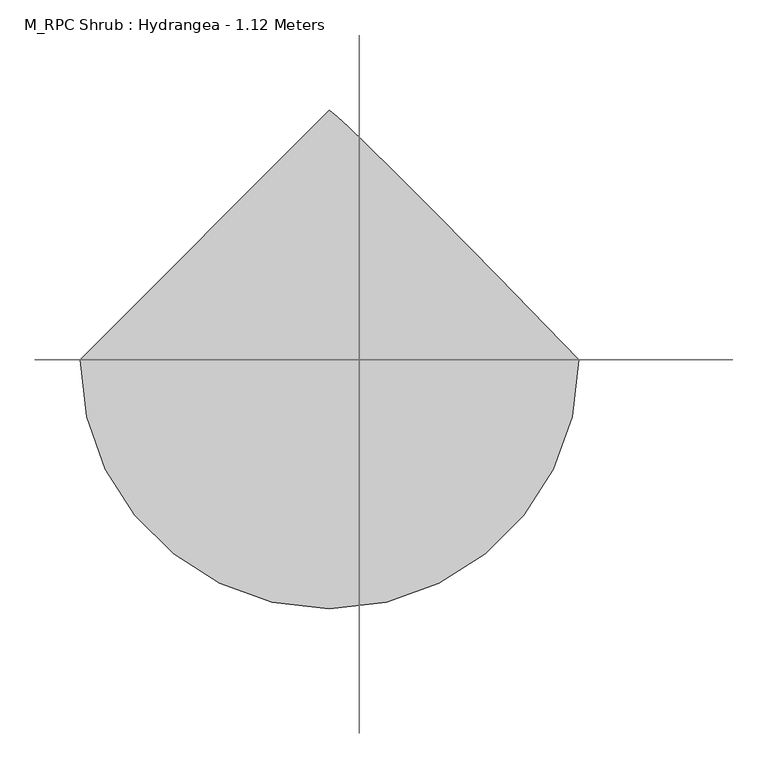
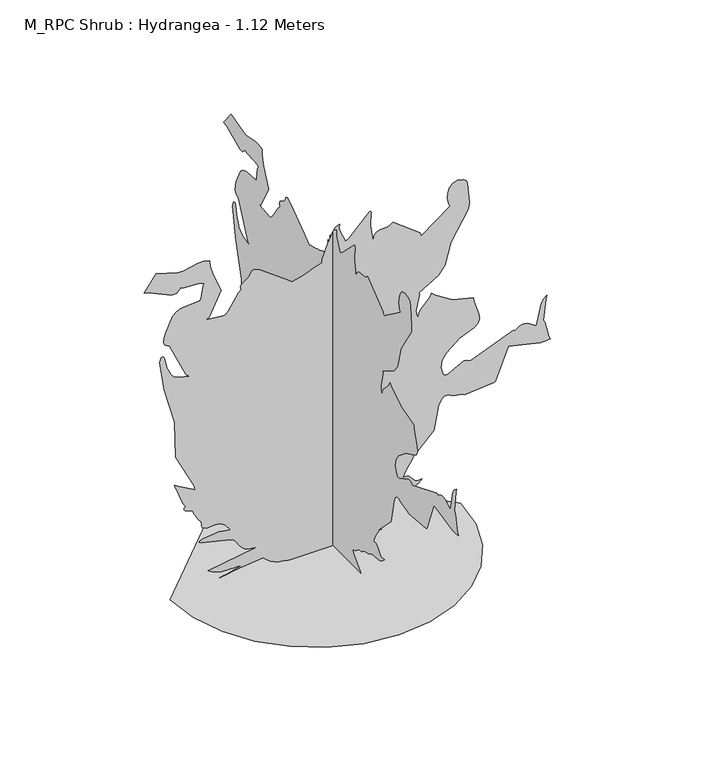
"""IFC4 building model written with IfcOpenShell, lengths in millimetres: geographic element geometry, M_RPC Shrub : Hydrangea - 1.12 Meters."""

from ifc_helpers import new_model, si_unit, origin, place, context, project, spatial, triangles, source, transform, mapped, element, save


def m_rpc_shrub_hydrangea_1_12_meters_e26dcdf9(model_context):
    return source(origin(), model_context, "Body", "Tessellation", [
        triangles([(-465.7652839, 0.0, 3.03e-05), (-453.4503742, -106.722383, 3.03e-05), (-418.3841643, -204.7301452, 3.03e-05), (-363.3691721, -291.2156366, 3.03e-05), (-291.2156366, -363.3691721, 3.03e-05), (-204.7298909, -418.3841643, 3.03e-05), (-106.722383, -453.4503742, 3.03e-05), (2.04e-05, -465.7652839, 3.03e-05), (106.7226373, -453.4503742, 3.03e-05), (204.7301452, -418.3841643, 3.03e-05), (291.2156366, -363.3691721, 3.03e-05), (363.3691721, -291.2156366, 3.03e-05), (418.3841643, -204.7298909, 3.03e-05), (453.4503742, -106.722383, 3.03e-05), (465.7652839, 4.07e-05, 3.03e-05), (314.4022119, 155.2617258, 3.03e-05), (202.1882401, 269.5741523, 3.03e-05), (122.6004381, 349.7611364, 3.03e-05), (69.1127373, 402.650677, 3.03e-05), (35.2001157, 435.0619981, 3.03e-05), (14.3374424, 453.8270954, 3.03e-05), (-6.11e-05, 465.7652839, 3.03e-05), (56.1492344, -378.5859032, 896.584009), (56.1492344, -435.8001798, 990.1474113), (56.1492344, -437.9638195, 1010.0427086), (56.1492344, -432.6209044, 1076.3849527), (56.1492344, -428.4870724, 1086.8671618), (56.1492344, -421.1205162, 1093.7984247), (56.1492344, -400.1306637, 1098.3878975), (56.1492344, -384.9139326, 1093.7296789), (56.1492344, -374.9204656, 1082.3183842), (56.1492344, -369.6029849, 1066.6409254), (56.1492344, -368.4091624, 1049.1918451), (56.1492344, -370.7917205, 1032.4579828), (56.1492344, -376.200838, 1018.9314102), (56.1492344, -284.4905202, 951.5531828), (56.1492344, -279.0483378, 962.8982752), (56.1492344, -192.4284615, 1029.6936167), (56.1492344, -183.9065071, 1021.5888788), (56.1492344, -173.6880356, 1018.7583103), (56.1492344, -151.8174592, 1018.2594309), (56.1492344, -141.9947939, 1015.253219), (56.1492344, -134.1316202, 1006.853223), (56.1492344, -129.1432891, 990.3891844), (56.1492344, -120.5388725, 1040.242028), (56.1492344, -122.2206557, 1090.0057056), (56.1492344, -121.588872, 1091.2198757), (56.1492344, -120.5788409, 1091.6016838), (56.1492344, -119.3498916, 1091.314056), (56.1492344, -118.0631606, 1090.5223892), (56.1492344, -51.1270437, 1024.7248793), (56.1492344, -40.2401219, 1017.5288795), (56.1492344, -21.4382513, 1061.8860558), (56.1492344, -19.9459255, 1071.2685499), (56.1492344, -20.5882464, 1082.5678602), (56.1492344, -9.2161605, 1076.7642174), (56.1492344, -0.541737, 1066.0147282), (56.1492344, 13.2312884, 1034.0107224), (56.1492344, 15.0516987, 1033.3972424), (56.1492344, 16.1430633, 1042.7950699), (56.1492344, 15.8630375, 1032.315477), (56.1492344, 35.0076788, 982.2768162), (56.1492344, 34.7279334, 971.7971506), (56.1492344, 47.0023863, 967.7320644), (56.1492344, 59.9819265, 963.0433245), (56.1492344, 73.5461604, 958.0542395), (56.1492344, 87.5764677, 953.090589), (56.1492344, 101.9527068, 948.4782251), (56.1492344, 116.5559942, 944.5379133), (56.1492344, 131.266706, 941.5953604), (56.1492344, 159.1710257, 963.3564594), (56.1492344, 234.8070158, 1017.7426746), (56.1492344, 253.0856966, 1025.9415928), (56.1492344, 261.255583, 1022.6172318), (56.1492344, 265.0508637, 1010.9616205), (56.1492344, 271.5392395, 1003.587434), (56.1492344, 292.8116329, 989.8291895), (56.1492344, 295.7185412, 982.2462948), (56.1492344, 294.1403672, 970.2699183), (56.1492344, 302.2043736, 963.0229769), (56.1492344, 334.2949656, 913.7683525), (56.1492344, 342.6898747, 905.5160219), (56.1492344, 351.4004259, 902.5404041), (56.1492344, 406.148138, 908.504357), (56.1492344, 397.9441329, 914.2774784), (56.1492344, 358.0695319, 991.6771872), (56.1492344, 384.2062723, 1053.5038639), (56.1492344, 393.7135772, 1085.5969631), (56.1492344, 394.9175735, 1105.0289892), (56.1492344, 414.6906761, 1109.8475178), (56.1492344, 432.1779808, 1109.2748056), (56.1492344, 480.121675, 1098.4515564), (56.1492344, 497.6624285, 1099.5588289), (56.1492344, 567.1076082, 1120.0013311), (56.1492344, 606.4145476, 1067.5955183), (56.1492344, 591.7069061, 1065.4878708), (56.1492344, 517.0715272, 1030.4623198), (56.1492344, 500.9715288, 1032.2518181), (56.1492344, 488.49878, 1045.1369328), (56.1492344, 477.9249341, 1041.5376612), (56.1492344, 432.2085385, 1040.0638412), (56.1492344, 422.1870572, 1037.8874479), (56.1492344, 413.6343089, 1032.9696522), (56.1492344, 417.3048697, 1026.0867147), (56.1492344, 423.0626942, 986.5124588), (56.1492344, 426.7357985, 979.6269779), (56.1492344, 479.2129369, 976.8397207), (56.1492344, 491.6474977, 973.836125), (56.1492344, 503.2929714, 967.8211578), (56.1492344, 513.8846214, 957.7538944), (56.1492344, 537.5548336, 908.2956488), (56.1492344, 541.9203012, 892.3381926), (56.1492344, 542.610121, 878.2821465), (56.1492344, 538.0995678, 867.797394), (56.1492344, 524.5653648, 859.2141243), (56.1492344, 471.3347477, 744.5693052), (56.1492344, 460.1321975, 735.9044998), (56.1492344, 496.5424387, 744.6049135), (56.1492344, 507.3555141, 749.4158117), (56.1492344, 516.4402794, 756.3470747), (56.1492344, 523.1577473, 766.0961889), (56.1492344, 526.8690033, 779.3631117), (56.1492344, 532.2882946, 786.419149), (56.1492344, 540.9835851, 826.8283104), (56.1492344, 544.9977659, 831.6620996), (56.1492344, 551.7839433, 831.0664965), (56.1492344, 556.8366872, 815.0530117), (56.1492344, 541.9737499, 718.1015894), (56.1492344, 508.528989, 595.9425488), (56.1492344, 504.1736953, 476.8583931), (56.1492344, 445.00198, 359.8157189), (56.1492344, 442.0517967, 344.7389503), (56.1492344, 498.367509, 375.5670104), (56.1492344, 507.2155154, 382.5721061), (56.1492344, 508.4017076, 380.6935507), (56.1492344, 480.3736945, 310.0265705), (56.1492344, 472.5896856, 298.8163718), (56.1492344, 477.8714853, 294.0410819), (56.1492344, 477.8587681, 289.3930734), (56.1492344, 474.0736794, 285.1268912), (56.1492344, 461.2776581, 278.7937931), (56.1492344, 455.3060022, 277.2436152), (56.1492344, 451.6507384, 277.1188771), (56.1492344, 448.9347342, 271.42215), (56.1492344, 446.3994601, 265.944323), (56.1492344, 443.8616426, 260.5352237), (56.1492344, 441.1354646, 255.0446795), (56.1492344, 438.0401593, 249.3240076), (56.1492344, 434.3950693, 243.2202559), (56.1492344, 430.0117976, 236.5850141), (56.1492344, 424.8445258, 231.9143507), (56.1492344, 422.1564995, 227.0286025), (56.1492344, 421.13069, 222.1354782), (56.1492344, 420.9550467, 217.4424143), (56.1492344, 420.8125045, 213.1568838), (56.1492344, 419.8910491, 209.4863229), (56.1492344, 417.376159, 206.6384771), (56.1492344, 405.2165088, 201.5623153), (56.1492344, 393.8230182, 201.2377712), (56.1492344, 382.6001204, 202.7596986), (56.1492344, 370.95719, 203.2227154), (56.1492344, 358.2935371, 199.7216937), (56.1492344, 344.018609, 189.3512511), (56.1492344, 327.5393097, 169.2057329), (56.1492344, 364.5146327, 175.1936668), (56.1492344, 416.1365181, 169.3225681), (56.1492344, 425.6743443, 165.5346816), (56.1492344, 428.6066872, 161.7190351), (56.1492344, 423.5107046, 158.722016), (56.1492344, 327.5393097, 135.5160923), (56.1492344, 317.0469269, 128.8205254), (56.1492344, 309.0694705, 119.4107255), (56.1492344, 301.848, 108.7037664), (56.1492344, 293.6134553, 98.116195), (56.1492344, 282.5992476, 89.0650578), (56.1492344, 267.0465086, 82.9669016), (56.1492344, 245.1858699, 81.2382826), (56.1492344, 400.5328557, 55.0353398), (56.1492344, 387.9633831, 46.5487848), (56.1492344, 359.4237007, 37.5090999), (56.1492344, 291.9767275, 36.3188451), (56.1492344, 338.6400493, 23.9801451), (56.1492344, 350.1684154, 21.3613778), (56.1492344, 363.0993484, 18.5382114), (56.1492344, 356.3946342, 19.4966274), (56.1492344, 339.2585798, 22.5081329), (56.1492344, 315.3211238, 26.7056692), (56.1492344, 224.2112962, 38.0176831), (56.1492344, 212.000995, 26.2095603), (56.1492344, 199.2024303, 17.3446467), (56.1492344, 185.91387, 10.9324609), (56.1492344, 172.2333097, 6.482364), (56.1492344, 158.2584905, 3.5041026), (56.1492344, 144.0879256, 1.5067812), (56.1492344, 129.8191018, 0.0), (56.1492344, -156.6362603, 8.5e-06), (56.1492344, -151.989787, 6.9042229), (56.1492344, -116.5554855, 39.0040464), (56.1492344, -111.7351584, 47.433074), (56.1492344, -111.8306104, 55.7371229), (56.1492344, -119.5942535, 57.0004315), (56.1492344, -125.4931031, 59.6629825), (56.1492344, -130.4834689, 63.2543694), (56.1492344, -135.5219514, 67.303936), (56.1492344, -141.5656232, 71.3410306), (56.1492344, -149.5703308, 74.8950015), (56.1492344, -160.4934013, 77.495188), (56.1492344, -169.3279093, 84.1324646), (56.1492344, -176.9146555, 87.7419281), (56.1492344, -197.1803154, 92.5151651), (56.1492344, -204.7667891, 96.1246287), (56.1492344, -213.6013152, 102.7621596), (56.1492344, -254.9555861, 106.7974783), (56.1492344, -265.9086966, 110.2895889), (56.1492344, -276.3806954, 116.5285068), (56.1492344, -286.0101585, 126.3919036), (56.1492344, -271.3101474, 125.9887033), (56.1492344, -261.5992212, 129.8282673), (56.1492344, -244.5843623, 149.5728742), (56.1492344, -237.0167283, 153.1530609), (56.1492344, -225.533145, 152.3609126), (56.1492344, -235.0936262, 173.0333336), (56.1492344, -246.7467303, 193.6841261), (56.1492344, -260.1330498, 213.7614254), (56.1492344, -323.7949525, 277.291977), (56.1492344, -338.7825914, 355.3942592), (56.1492344, -346.347682, 371.8098996), (56.1492344, -357.0004475, 381.6099192), (56.1492344, -371.5222718, 382.1062915), (56.1492344, -376.9797149, 377.4022908), (56.1492344, -383.7735589, 374.7193514), (56.1492344, -415.3219603, 368.8724336), (56.1492344, -422.0546888, 364.7920867), (56.1492344, -517.7944482, 372.8866508), (56.1492344, -522.1878937, 375.0858988), (56.1492344, -562.8388644, 478.6987604), (56.1492344, -664.7386402, 455.7362085), (56.1492344, -684.4684679, 455.2372928), (56.1492344, -698.1222857, 457.4391206), (56.1492344, -692.9499269, 465.9613111), (56.1492344, -680.8361315, 520.039551), (56.1492344, -675.6637001, 528.5617415), (56.1492344, -683.1117193, 596.1996188), (56.1492344, -686.8942646, 608.1072859), (56.1492344, -676.4070414, 599.0174701), (56.1492344, -668.8648418, 588.3647046), (56.1492344, -653.2051872, 517.331177), (56.1492344, -624.8614958, 535.1442976), (56.1492344, -615.2854815, 537.4631968), (56.1492344, -605.3836513, 536.9337596), (56.1492344, -594.9930791, 532.9272091), (56.1492344, -583.953455, 524.8173843), (56.1492344, -578.7047201, 528.4293732), (56.1492344, -441.3543466, 473.0096818), (56.1492344, -430.6838133, 478.8311288), (56.1492344, -420.9245253, 480.0758566), (56.1492344, -368.722261, 452.5772807), (56.1492344, -359.298999, 451.355444), (56.1492344, -354.0909957, 457.9074786), (56.1492344, -346.5386224, 482.3693213), (56.1492344, -350.8200471, 505.2580768), (56.1492344, -364.1684329, 526.1333651), (56.1492344, -407.0059344, 560.1203167), (56.1492344, -452.9285674, 580.8606932), (56.1492344, -466.1674759, 590.2839915), (56.1492344, -470.6474713, 604.2992698), (56.1492344, -468.9191248, 621.1578701), (56.1492344, -452.0605608, 671.2982689), (56.1492344, -451.0652727, 682.0375843), (56.1492344, -383.8320946, 699.9016102), (56.1492344, -330.0313087, 733.2954294), (56.1492344, -317.2429178, 745.2056036), (56.1492344, -312.1825799, 733.1910753), (56.1492344, -281.2959841, 701.540827), (56.1492344, -275.8410663, 691.562657), (56.1492344, -273.2599739, 678.2931908), (56.1492344, -267.5454244, 690.5215868), (56.1492344, -266.4457822, 704.0710505), (56.1492344, -277.6788902, 753.9034739), (56.1492344, -276.770152, 760.8805916), (56.1492344, -338.7673307, 798.0773037), (56.1492344, -359.6069744, 825.2042816), (434.7336388, 5.26e-05, 896.584009), (491.947879, 6.22e-05, 990.1474113), (494.1140622, 6.4e-05, 1010.0427086), (488.7711471, 6.94e-05, 1076.3849527), (484.6373151, 7.02e-05, 1086.8671618), (477.2682155, 7.05e-05, 1093.7984247), (456.2783629, 7.03e-05, 1098.3878975), (441.0616319, 6.95e-05, 1093.7296789), (431.0707083, 6.82e-05, 1082.3183842), (425.7506842, 6.67e-05, 1066.6409254), (424.5594415, 6.52e-05, 1049.1918451), (426.9419632, 6.39e-05, 1032.4579828), (432.3510807, 6.29e-05, 1018.9314102), (340.6382195, 5.45e-05, 951.5531828), (335.1960371, 5.53e-05, 962.8982752), (248.5774325, 5.84e-05, 1029.6936167), (240.0557506, 5.74e-05, 1021.5888788), (229.837261, 5.69e-05, 1018.7583103), (207.9666846, 5.62e-05, 1018.2594309), (198.143774, 5.56e-05, 1015.253219), (190.2808455, 5.47e-05, 1006.853223), (185.2922692, 5.32e-05, 990.3891844), (176.6878525, 5.67e-05, 1040.242028), (178.3696358, 6.12e-05, 1090.0057056), (177.7381155, 6.12e-05, 1091.2198757), (176.727821, 6.11e-05, 1091.6016838), (175.4988626, 6.1e-05, 1091.314056), (174.2123859, 6.09e-05, 1090.5223892), (107.2762736, 5.37e-05, 1024.7248793), (96.3893563, 5.28e-05, 1017.5288795), (77.5873336, 5.6e-05, 1061.8860558), (76.0951826, 5.67e-05, 1071.2685499), (76.7374036, 5.77e-05, 1082.5678602), (65.3653143, 5.69e-05, 1076.7642174), (56.6909074, 5.56e-05, 1066.0147282), (42.9179427, 5.25e-05, 1034.0107224), (41.0974324, 5.24e-05, 1033.3972424), (40.0061927, 5.32e-05, 1042.7950699), (40.2861947, 5.23e-05, 1032.315477), (21.1414012, 4.76e-05, 982.2768162), (21.4212988, 4.67e-05, 971.7971506), (9.1466437, 4.6e-05, 967.7320644), (-3.8326703, 4.52e-05, 963.0433245), (-17.3969816, 4.44e-05, 958.0542395), (-31.4272378, 4.35e-05, 953.090589), (-45.8034724, 4.27e-05, 948.4782251), (-60.4067643, 4.19e-05, 944.5379133), (-75.1174716, 4.12e-05, 941.5953604), (-103.0218003, 4.22e-05, 963.3564594), (-178.6577904, 4.46e-05, 1017.7426746), (-196.9364531, 4.47e-05, 1025.9415928), (-205.1063577, 4.42e-05, 1022.6172318), (-208.9011297, 4.31e-05, 1010.9616205), (-215.3900142, 4.23e-05, 1003.587434), (-236.6618807, 4.05e-05, 989.8291895), (-239.5693159, 3.98e-05, 982.2462948), (-237.9918868, 3.88e-05, 970.2699183), (-246.0546214, 3.8e-05, 963.0229769), (-278.1447048, 3.29e-05, 913.7683525), (-286.5421755, 3.19e-05, 905.5160219), (-295.2527267, 3.14e-05, 902.5404041), (-349.9978952, 3.03e-05, 908.504357), (-341.7964336, 3.1e-05, 914.2774784), (-301.919271, 3.87e-05, 991.6771872), (-328.0560296, 4.32e-05, 1053.5038639), (-337.5633345, 4.56e-05, 1085.5969631), (-338.7673307, 4.72e-05, 1105.0289892), (-358.5404334, 4.7e-05, 1109.8475178), (-376.0302815, 4.64e-05, 1109.2748056), (-423.9739758, 4.41e-05, 1098.4515564), (-441.5121858, 4.37e-05, 1099.5588289), (-510.959909, 4.33e-05, 1120.0013311), (-550.2643049, 3.77e-05, 1067.5955183), (-535.5592069, 3.8e-05, 1065.4878708), (-460.9238279, 3.73e-05, 1030.4623198), (-444.8238296, 3.79e-05, 1032.2518181), (-432.3510807, 3.93e-05, 1045.1369328), (-421.7772348, 3.93e-05, 1041.5376612), (-376.0582595, 4.06e-05, 1040.0638412), (-366.0368145, 4.07e-05, 1037.8874479), (-357.4840662, 4.05e-05, 1032.9696522), (-361.1571705, 3.98e-05, 1026.0867147), (-366.9149949, 3.63e-05, 986.5124588), (-370.5855557, 3.56e-05, 979.6269779), (-423.0652376, 3.39e-05, 976.8397207), (-435.4997984, 3.33e-05, 973.836125), (-447.1427287, 3.24e-05, 967.8211578), (-457.7343787, 3.13e-05, 957.7538944), (-481.4045909, 2.64e-05, 908.2956488), (-485.7700584, 2.48e-05, 892.3381926), (-486.4598783, 2.37e-05, 878.2821465), (-481.9493251, 2.29e-05, 867.797394), (-468.4176656, 2.26e-05, 859.2141243), (-415.184505, 1.45e-05, 744.5693052), (-403.9844982, 1.41e-05, 735.9044998), (-440.3921597, 1.37e-05, 744.6049135), (-451.2052714, 1.39e-05, 749.4158117), (-460.2900003, 1.42e-05, 756.3470747), (-467.0074682, 1.48e-05, 766.0961889), (-470.7187606, 1.58e-05, 779.3631117), (-476.1380519, 1.63e-05, 786.419149), (-484.833306, 1.94e-05, 826.8283104), (-488.8475232, 1.96e-05, 831.6620996), (-495.636244, 1.94e-05, 831.0664965), (-500.6889879, 1.79e-05, 815.0530117), (-485.8235072, 1.02e-05, 718.1015894), (-452.3812898, 9e-07, 595.9425488), (-448.025996, -9e-06, 476.8583931), (-388.8542808, -1.71e-05, 359.8157189), (-385.901554, -1.83e-05, 344.7389503), (-442.2198097, -1.74e-05, 375.5670104), (-451.0678162, -1.71e-05, 382.5721061), (-452.2540083, -1.74e-05, 380.6935507), (-424.2234155, -2.24e-05, 310.0265705), (-416.44195, -2.31e-05, 298.8163718), (-421.7212426, -2.37e-05, 294.0410819), (-421.7085254, -2.4e-05, 289.3930734), (-417.9259801, -2.42e-05, 285.1268912), (-405.1274154, -2.43e-05, 278.7937931), (-399.158303, -2.43e-05, 277.2436152), (-395.5030392, -2.43e-05, 277.1188771), (-392.7870349, -2.47e-05, 271.42215), (-390.2492174, -2.5e-05, 265.944323), (-387.7113999, -2.55e-05, 260.5352237), (-384.9851855, -2.59e-05, 255.0446795), (-381.8924601, -2.62e-05, 249.3240076), (-378.2448266, -2.66e-05, 243.2202559), (-373.8615549, -2.7e-05, 236.5850141), (-368.6968266, -2.73e-05, 231.9143507), (-366.0062568, -2.76e-05, 227.0286025), (-364.9804473, -2.8e-05, 222.1354782), (-364.8048039, -2.84e-05, 217.4424143), (-364.6622618, -2.87e-05, 213.1568838), (-363.7408064, -2.91e-05, 209.4863229), (-361.2284234, -2.92e-05, 206.6384771), (-349.0687732, -2.93e-05, 201.5623153), (-337.6727755, -2.9e-05, 201.2377712), (-326.4523848, -2.85e-05, 202.7596986), (-314.8069473, -2.81e-05, 203.2227154), (-302.1458197, -2.8e-05, 199.7216937), (-287.8708916, -2.85e-05, 189.3512511), (-271.389067, -2.97e-05, 169.2057329), (-308.36439, -3.01e-05, 175.1936668), (-359.9888188, -3.18e-05, 169.3225681), (-369.5241016, -3.25e-05, 165.5346816), (-372.4564445, -3.33e-05, 161.7190351), (-367.3604619, -3.31e-05, 158.722016), (-271.389067, -3.25e-05, 135.5160923), (-260.8966842, -3.28e-05, 128.8205254), (-252.9212626, -3.33e-05, 119.4107255), (-245.6982659, -3.4e-05, 108.7037664), (-237.4631945, -3.47e-05, 98.116195), (-226.4505309, -3.51e-05, 89.0650578), (-210.8967746, -3.51e-05, 82.9669016), (-189.0366264, -3.46e-05, 81.2382826), (-344.382613, -4.15e-05, 55.0353398), (-331.8131404, -4.16e-05, 46.5487848), (-303.273458, -4.15e-05, 37.5090999), (-235.827484, -3.98e-05, 36.3188451), (-282.49235, -4.22e-05, 23.9801701), (-294.0207161, -4.28e-05, 21.3614051), (-306.9491057, -4.34e-05, 18.5382375), (-300.2443733, -4.32e-05, 19.4966524), (-283.1083371, -4.24e-05, 22.5081578), (-259.1734064, -4.14e-05, 26.7056692), (-168.0623071, -3.77e-05, 38.0176831), (-155.8517515, -3.83e-05, 26.2095603), (-143.0531959, -3.87e-05, 17.3446467), (-129.7646356, -3.88e-05, 10.9324859), (-116.0840662, -3.88e-05, 6.482364), (-102.1092561, -3.86e-05, 3.5041278), (-87.9386912, -3.83e-05, 1.5067912), (-73.6701263, -3.81e-05, 9.3e-06), (212.7852495, -2.96e-05, 5.3e-06), (208.1390214, -2.91e-05, 6.9042229), (172.7047199, -2.74e-05, 39.0040464), (167.8843928, -2.69e-05, 47.433074), (167.9795905, -2.62e-05, 55.7371229), (175.7434879, -2.59e-05, 57.0004315), (181.6420741, -2.54e-05, 59.6629825), (186.632449, -2.5e-05, 63.2543694), (191.6709314, -2.45e-05, 67.303936), (197.7148576, -2.4e-05, 71.3410306), (205.7195652, -2.34e-05, 74.8950015), (216.6423723, -2.29e-05, 77.495188), (225.4768985, -2.2e-05, 84.1324646), (233.0636265, -2.15e-05, 87.7419281), (253.3292863, -2.05e-05, 92.5151651), (260.9170499, -2e-05, 96.1246287), (269.7497775, -1.91e-05, 102.7621596), (311.1032853, -1.76e-05, 106.7974783), (322.0589393, -1.69e-05, 110.2893346), (332.5309381, -1.61e-05, 116.5285068), (342.1604012, -1.5e-05, 126.3919036), (327.4603901, -1.55e-05, 125.9887033), (317.7469205, -1.54e-05, 129.8282673), (300.7330971, -1.43e-05, 149.5728742), (293.1654449, -1.42e-05, 153.1530609), (281.6828972, -1.46e-05, 152.3609126), (291.2436327, -1.26e-05, 173.0333336), (302.8967368, -1.05e-05, 193.6841261), (316.2807673, -8.4e-06, 213.7614254), (379.9426517, -1.2e-06, 277.291977), (394.9302907, 5.8e-06, 355.3942592), (402.4954176, 7.5e-06, 371.8098996), (413.1481467, 8.6e-06, 381.6099192), (427.6699711, 9.1e-06, 382.1062915), (433.1274505, 8.8e-06, 377.4022908), (439.9212582, 8.8e-06, 374.7193514), (471.472203, 9.3e-06, 368.8724336), (478.2049315, 9.2e-06, 364.7920867), (573.9446909, 1.26e-05, 372.8866508), (578.3381727, 1.3e-05, 375.0858988), (618.9865637, 2.29e-05, 478.6987604), (720.8863031, 2.4e-05, 455.7362085), (740.6162035, 2.46e-05, 455.2372928), (754.2725647, 2.52e-05, 457.4391206), (749.100206, 2.57e-05, 465.9613111), (736.9863379, 2.99e-05, 520.039551), (731.8139791, 3.05e-05, 528.5617415), (739.2619984, 3.64e-05, 596.1996188), (743.0420002, 3.75e-05, 608.1072859), (732.5572477, 3.65e-05, 599.0174701), (725.0150482, 3.53e-05, 588.3647046), (709.3528502, 2.89e-05, 517.331177), (681.0091587, 2.96e-05, 535.1442976), (671.4357605, 2.94e-05, 537.4631968), (661.533894, 2.91e-05, 536.9337596), (651.1407784, 2.85e-05, 532.9272091), (640.1011179, 2.74e-05, 524.8173843), (634.852383, 2.76e-05, 528.4293732), (497.5020458, 1.88e-05, 473.0096818), (486.8315125, 1.9e-05, 478.8311288), (477.074768, 1.88e-05, 480.0758566), (424.8725038, 1.49e-05, 452.5772807), (415.4466983, 1.46e-05, 451.355444), (410.2412384, 1.49e-05, 457.9074786), (402.6888651, 1.72e-05, 482.3693213), (406.9703261, 1.95e-05, 505.2580768), (420.3187119, 2.16e-05, 526.1333651), (463.1562135, 2.54e-05, 560.1203167), (509.0762667, 2.82e-05, 580.8606932), (522.3177186, 2.94e-05, 590.2839915), (526.7951706, 3.07e-05, 604.2992698), (525.0693675, 3.21e-05, 621.1578701), (508.2082601, 3.59e-05, 671.2982689), (507.2155154, 3.67e-05, 682.0375843), (439.9797938, 3.63e-05, 699.9016102), (386.179008, 3.75e-05, 733.2954294), (373.3931969, 3.81e-05, 745.2056036), (368.3302792, 3.69e-05, 733.1910753), (337.4462268, 3.33e-05, 701.540827), (331.9887837, 3.23e-05, 691.562657), (329.4102347, 3.11e-05, 678.2931908), (323.6956853, 3.2e-05, 690.5215868), (322.5934997, 3.31e-05, 704.0710505), (333.8265713, 3.77e-05, 753.9034739), (332.9178695, 3.82e-05, 760.8805916), (394.9175735, 4.32e-05, 798.0773037), (415.7572171, 4.61e-05, 825.2042816)], [[21, 22, 1], [20, 21, 1], [19, 20, 1], [18, 19, 1], [17, 18, 1], [17, 1, 2], [17, 2, 3], [17, 3, 4], [16, 17, 4], [16, 4, 5], [16, 5, 6], [16, 6, 7], [16, 7, 8], [16, 8, 9], [16, 9, 10], [16, 10, 11], [16, 11, 12], [15, 16, 12], [14, 15, 12], [13, 14, 12], [183, 184, 185], [59, 60, 61], [183, 185, 186], [182, 183, 186], [243, 244, 245], [177, 178, 179], [215, 216, 217], [195, 196, 197], [195, 197, 198], [182, 186, 187], [181, 182, 187], [181, 187, 188], [54, 55, 56], [94, 95, 96], [238, 239, 240], [195, 198, 199], [271, 272, 273], [167, 168, 169], [133, 134, 135], [214, 215, 217], [214, 217, 218], [177, 179, 180], [177, 180, 181], [166, 167, 169], [165, 166, 169], [164, 165, 169], [164, 169, 170], [37, 38, 39], [213, 214, 218], [94, 96, 97], [93, 94, 97], [93, 97, 98], [93, 98, 99], [92, 93, 99], [92, 99, 100], [92, 100, 101], [91, 92, 101], [90, 91, 101], [90, 101, 102], [89, 90, 102], [88, 89, 102], [87, 88, 102], [87, 102, 103], [195, 199, 200], [54, 56, 57], [53, 54, 57], [243, 245, 246], [242, 243, 246], [242, 246, 247], [241, 242, 247], [268, 269, 270], [87, 103, 104], [86, 87, 104], [86, 104, 105], [86, 105, 106], [85, 86, 106], [84, 85, 106], [133, 135, 136], [132, 133, 136], [132, 136, 137], [53, 57, 58], [125, 126, 127], [124, 125, 127], [123, 124, 127], [123, 127, 128], [122, 123, 128], [121, 122, 128], [120, 121, 128], [119, 120, 128], [52, 53, 58], [177, 181, 188], [118, 119, 128], [213, 218, 219], [213, 219, 220], [213, 220, 221], [212, 213, 221], [117, 118, 128], [164, 170, 171], [237, 238, 240], [237, 240, 241], [237, 241, 247], [237, 247, 248], [237, 248, 249], [237, 249, 250], [237, 250, 251], [237, 251, 252], [236, 237, 252], [236, 252, 253], [236, 253, 254], [235, 236, 254], [234, 235, 254], [233, 234, 254], [232, 233, 254], [232, 254, 255], [232, 255, 256], [232, 256, 257], [231, 232, 257], [230, 231, 257], [229, 230, 257], [229, 257, 258], [228, 229, 258], [84, 106, 107], [84, 107, 108], [84, 108, 109], [84, 109, 110], [84, 110, 111], [84, 111, 112], [84, 112, 113], [84, 113, 114], [84, 114, 115], [84, 115, 116], [84, 116, 117], [83, 84, 117], [270, 271, 273], [73, 74, 75], [72, 73, 75], [137, 138, 139], [137, 139, 140], [137, 140, 141], [132, 137, 141], [132, 141, 142], [132, 142, 143], [72, 75, 76], [227, 228, 258], [227, 258, 259], [117, 128, 129], [224, 225, 226], [46, 47, 48], [46, 48, 49], [46, 49, 50], [45, 46, 50], [45, 50, 51], [44, 45, 51], [44, 51, 52], [211, 212, 221], [210, 211, 221], [209, 210, 221], [82, 83, 117], [270, 273, 274], [270, 274, 275], [270, 275, 276], [264, 265, 266], [264, 266, 267], [264, 267, 268], [264, 268, 270], [263, 264, 270], [263, 270, 276], [262, 263, 276], [261, 262, 276], [52, 58, 59], [52, 59, 61], [52, 61, 62], [52, 62, 63], [44, 52, 63], [260, 261, 276], [71, 72, 76], [71, 76, 77], [71, 77, 78], [71, 78, 79], [71, 79, 80], [70, 71, 80], [70, 80, 81], [70, 81, 82], [70, 82, 117], [70, 117, 129], [70, 129, 130], [70, 130, 131], [69, 70, 131], [68, 69, 131], [67, 68, 131], [67, 131, 132], [66, 67, 132], [65, 66, 132], [64, 65, 132], [63, 64, 132], [44, 63, 132], [132, 143, 144], [44, 132, 144], [44, 144, 145], [44, 145, 146], [44, 146, 147], [44, 147, 148], [44, 148, 149], [44, 149, 150], [44, 150, 151], [44, 151, 152], [44, 152, 153], [44, 153, 154], [44, 154, 155], [44, 155, 156], [44, 156, 157], [44, 157, 158], [44, 158, 159], [44, 159, 160], [44, 160, 161], [44, 161, 162], [44, 162, 163], [44, 163, 164], [44, 164, 171], [44, 171, 172], [44, 172, 173], [44, 173, 174], [44, 174, 175], [44, 175, 176], [44, 176, 177], [44, 177, 188], [44, 188, 189], [44, 189, 190], [44, 190, 191], [44, 191, 192], [44, 192, 193], [44, 193, 194], [44, 194, 195], [44, 195, 200], [44, 200, 201], [44, 201, 202], [44, 202, 203], [44, 203, 204], [44, 204, 205], [44, 205, 206], [44, 206, 207], [44, 207, 208], [44, 208, 209], [44, 209, 221], [44, 221, 222], [44, 222, 223], [44, 223, 224], [44, 224, 226], [44, 226, 227], [44, 227, 259], [44, 259, 260], [43, 44, 260], [42, 43, 260], [29, 30, 31], [28, 29, 31], [28, 31, 32], [27, 28, 32], [26, 27, 32], [26, 32, 33], [26, 33, 34], [26, 34, 35], [25, 26, 35], [24, 25, 35], [23, 24, 35], [23, 35, 36], [282, 23, 36], [281, 282, 36], [280, 281, 36], [37, 39, 40], [280, 36, 37], [280, 37, 40], [280, 40, 41], [280, 41, 42], [279, 280, 42], [278, 279, 42], [277, 278, 42], [277, 42, 260], [277, 260, 276], [443, 444, 445], [319, 320, 321], [443, 445, 446], [442, 443, 446], [503, 504, 505], [437, 438, 439], [475, 476, 477], [455, 456, 457], [455, 457, 458], [442, 446, 447], [441, 442, 447], [441, 447, 448], [314, 315, 316], [354, 355, 356], [498, 499, 500], [455, 458, 459], [531, 532, 533], [427, 428, 429], [393, 394, 395], [474, 475, 477], [474, 477, 478], [437, 439, 440], [437, 440, 441], [426, 427, 429], [425, 426, 429], [424, 425, 429], [424, 429, 430], [297, 298, 299], [473, 474, 478], [354, 356, 357], [353, 354, 357], [353, 357, 358], [353, 358, 359], [352, 353, 359], [352, 359, 360], [352, 360, 361], [351, 352, 361], [350, 351, 361], [350, 361, 362], [349, 350, 362], [348, 349, 362], [347, 348, 362], [347, 362, 363], [455, 459, 460], [314, 316, 317], [313, 314, 317], [503, 505, 506], [502, 503, 506], [502, 506, 507], [501, 502, 507], [528, 529, 530], [347, 363, 364], [346, 347, 364], [346, 364, 365], [346, 365, 366], [345, 346, 366], [344, 345, 366], [393, 395, 396], [392, 393, 396], [392, 396, 397], [313, 317, 318], [385, 386, 387], [384, 385, 387], [383, 384, 387], [383, 387, 388], [382, 383, 388], [381, 382, 388], [380, 381, 388], [379, 380, 388], [312, 313, 318], [437, 441, 448], [378, 379, 388], [473, 478, 479], [473, 479, 480], [473, 480, 481], [472, 473, 481], [377, 378, 388], [424, 430, 431], [497, 498, 500], [497, 500, 501], [497, 501, 507], [497, 507, 508], [497, 508, 509], [497, 509, 510], [497, 510, 511], [497, 511, 512], [496, 497, 512], [496, 512, 513], [496, 513, 514], [495, 496, 514], [494, 495, 514], [493, 494, 514], [492, 493, 514], [492, 514, 515], [492, 515, 516], [492, 516, 517], [491, 492, 517], [490, 491, 517], [489, 490, 517], [489, 517, 518], [488, 489, 518], [344, 366, 367], [344, 367, 368], [344, 368, 369], [344, 369, 370], [344, 370, 371], [344, 371, 372], [344, 372, 373], [344, 373, 374], [344, 374, 375], [344, 375, 376], [344, 376, 377], [343, 344, 377], [530, 531, 533], [333, 334, 335], [332, 333, 335], [397, 398, 399], [397, 399, 400], [397, 400, 401], [392, 397, 401], [392, 401, 402], [392, 402, 403], [332, 335, 336], [487, 488, 518], [487, 518, 519], [377, 388, 389], [484, 485, 486], [306, 307, 308], [306, 308, 309], [306, 309, 310], [305, 306, 310], [305, 310, 311], [304, 305, 311], [304, 311, 312], [471, 472, 481], [470, 471, 481], [469, 470, 481], [342, 343, 377], [530, 533, 534], [530, 534, 535], [530, 535, 536], [524, 525, 526], [524, 526, 527], [524, 527, 528], [524, 528, 530], [523, 524, 530], [523, 530, 536], [522, 523, 536], [521, 522, 536], [312, 318, 319], [312, 319, 321], [312, 321, 322], [312, 322, 323], [304, 312, 323], [520, 521, 536], [331, 332, 336], [331, 336, 337], [331, 337, 338], [331, 338, 339], [331, 339, 340], [330, 331, 340], [330, 340, 341], [330, 341, 342], [330, 342, 377], [330, 377, 389], [330, 389, 390], [330, 390, 391], [329, 330, 391], [328, 329, 391], [327, 328, 391], [327, 391, 392], [326, 327, 392], [325, 326, 392], [324, 325, 392], [323, 324, 392], [304, 323, 392], [392, 403, 404], [304, 392, 404], [304, 404, 405], [304, 405, 406], [304, 406, 407], [304, 407, 408], [304, 408, 409], [304, 409, 410], [304, 410, 411], [304, 411, 412], [304, 412, 413], [304, 413, 414], [304, 414, 415], [304, 415, 416], [304, 416, 417], [304, 417, 418], [304, 418, 419], [304, 419, 420], [304, 420, 421], [304, 421, 422], [304, 422, 423], [304, 423, 424], [304, 424, 431], [304, 431, 432], [304, 432, 433], [304, 433, 434], [304, 434, 435], [304, 435, 436], [304, 436, 437], [304, 437, 448], [304, 448, 449], [304, 449, 450], [304, 450, 451], [304, 451, 452], [304, 452, 453], [304, 453, 454], [304, 454, 455], [304, 455, 460], [304, 460, 461], [304, 461, 462], [304, 462, 463], [304, 463, 464], [304, 464, 465], [304, 465, 466], [304, 466, 467], [304, 467, 468], [304, 468, 469], [304, 469, 481], [304, 481, 482], [304, 482, 483], [304, 483, 484], [304, 484, 486], [304, 486, 487], [304, 487, 519], [304, 519, 520], [303, 304, 520], [302, 303, 520], [289, 290, 291], [288, 289, 291], [288, 291, 292], [287, 288, 292], [286, 287, 292], [286, 292, 293], [286, 293, 294], [286, 294, 295], [285, 286, 295], [284, 285, 295], [283, 284, 295], [283, 295, 296], [542, 283, 296], [541, 542, 296], [540, 541, 296], [297, 299, 300], [540, 296, 297], [540, 297, 300], [540, 300, 301], [540, 301, 302], [539, 540, 302], [538, 539, 302], [537, 538, 302], [537, 302, 520], [537, 520, 536]], closed=False),
    ])


if __name__ == "__main__":
    model = new_model("IFC4")
    model_context = context("Model", 3, world=origin())
    ifc_project = project(units=[si_unit("LENGTHUNIT", "METRE", prefix="MILLI")], contexts=[model_context])
    site = spatial("IfcSite", under=ifc_project)
    building = spatial("IfcBuilding", under=site)
    placement = place(None, origin())
    m_rpc_shrub_hydrangea_1_12_meters_shape = m_rpc_shrub_hydrangea_1_12_meters_e26dcdf9(model_context)
    element("IfcGeographicElement", 1, ObjectType="M_RPC Shrub : Hydrangea - 1.12 Meters", at=placement, inside=building, context=model_context, shape_type="MappedRepresentation", body=[
        mapped(m_rpc_shrub_hydrangea_1_12_meters_shape, transform((0.0, 0.0, 0.0), x_axis=(1.0, 0.0, 0.0), y_axis=(0.0, 1.0, 0.0), z_axis=(0.0, 0.0, 1.0))),
    ])
    save(model, "model.ifc")

# Revit data of these elements
# Type "M_RPC Shrub : Hydrangea - 1.12 Meters"
#   Type Comments = "Hydrangea"
#   built-in parameter 1005198 = "{2, 15},{39, RPC-16-FW46-UP80-R12G-Q000-ST1L-LVER-AU},{1, 0},{1, 0},{2, 35},{1, 8},{5, Color},{1, 0},{1, 0},{3, 0.8},{3, 0.8},{3, 0.8},{1, 8},{7, BBoxMin},{1, 0},{1, 0},{1, 0},{1, 0},{1, 0},{1, 8},{7, BBoxMax},{1, 0},{1, 0},{1, 0},{1, 0},{1, 0},{2, 11},{9, RPCTypeId},{1, 0},{1, 0},{39, RPC-16-FW46-UP80-R12G-Q000-ST1L-LVER-AU},{1, 6},{14, RPCPlantHeight},{1, 0},{1, 0},{7, 3.67454},{2, 11},{7, keyword},{1, 0},{1, 0},{23, :Geometry:RPC:Hydrangea},{2, 11},{8, category},{1, 0},{1, 0},{17, :Shrubs & Grasses},{2, 11},{12, LocalizedUID},{1, 0},{1, 0},{9, Hydrangea},{2, 14},{6, Height},{1, 0},{1, 0},{7, 3.67454},{1, 2},{16, Cast Reflections},{1, 0},{1, 0},{1, 0},{1, 2},{12, Cast Shadows},{1, 0},{1, 0},{1, 1},{1, 2},{9, Lock View},{1, 0},{1, 0},{1, 0},{1, 4},{5, ViewC},{1, 0},{1, 0},{1, 0},{2, 11},{20, AdvancedUIDefinition},{1, 0},{1, 0},{0, },{2, 11},{10, AssetLibID},{1, 0},{1, 0},{36, 4D3F6E72-3F99-4203-98E9-AF80B3C7A7A4},{2, 11},{10, BaseSchema},{1, 0},{1, 0},{9, RPCSchema},{2, 11},{12, ExchangeGUID},{1, 0},{1, 0},{0, },{1, 2},{6, Hidden},{1, 0},{1, 0},{1, 0},{1, 4},{11, RPCCategory},{1, 0},{1, 0},{1, 0},{2, 11},{8, RPCImage},{1, 0},{1, 0},{0, },{1, 4},{13, SchemaVersion},{1, 0},{1, 0},{1, 4},{2, 11},{12, UIDefinition},{1, 0},{1, 0},{0, },{2, 11},{6, UIName},{1, 0},{1, 0},{39, RPC-16-FW46-UP80-R12G-Q000-ST1L-LVER-AU},{2, 11},{11, VersionGUID},{1, 0},{1, 0},{9, RPCSchema},{2, 11},{9, assettype},{1, 0},{1, 0},{11, RPCGeometry},{2, 11},{11, description},{1, 0},{1, 0},{0, },{2, 11},{9, localname},{1, 0},{1, 0},{3, RPC},{2, 11},{9, localtype},{1, 0},{1, 0},{3, RPC},{1, 4},{8, revision},{1, 0},{1, 0},{1, 1},{2, 11},{9, thumbnail},{1, 0},{1, 0},{0, },{1, 4},{7, version},{1, 0},{1, 0},{1, 1},{1, 2},{20, RPC_Cast Reflections},{1, 0},{1, 0},{1, 1},{1, 2},{16, RPC_Cast Shadows},{1, 0},{1, 0},{1, 1},{1, 2},{13, RPC_Lock View},{1, 0},{1, 0},{1, 0},{1, 4},{9, RPC_ViewC},{1, 0},{1, 0},{1, 0},{21, assetlibrary_base.fbx},{1, 5},"
#   built-in parameter 1005195 = "RPC-16-FW46-UP80-R12G-Q000-ST1L-LVER-AU"
#   Height = 1.12 m
#   Description = (empty or 0)
#   Default Elevation = 0
